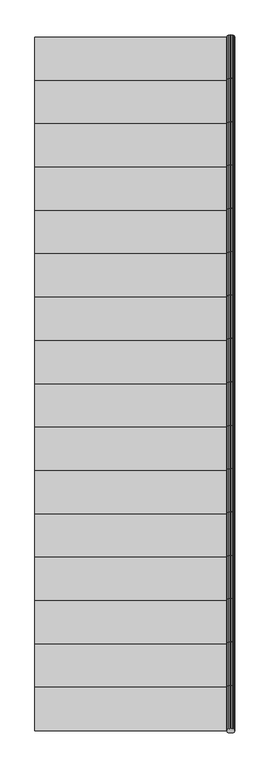
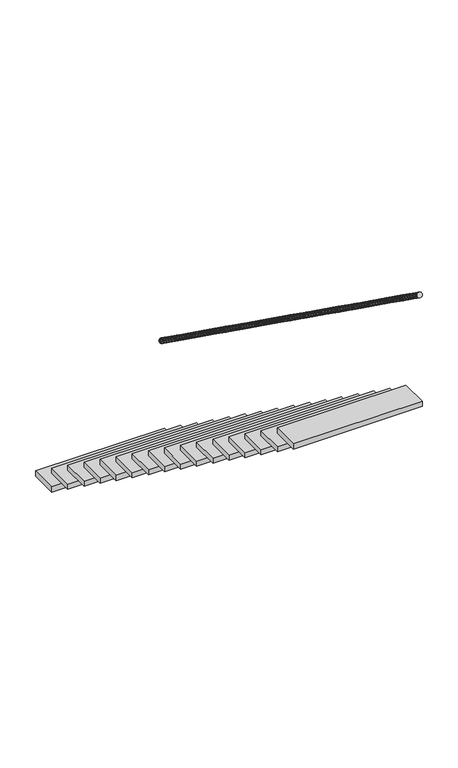
"""IFC4 building model written with IfcOpenShell, lengths in millimetres: stair geometry, 0_3d."""

from ifc_helpers import new_model, si_unit, frame, origin, origin_with_axes, place, context, project, spatial, polyline, outline, extrude, source, transform, mapped, element, save


def stair_085bacb0(model_context):
    return source(origin(), model_context, "Body", "SweptSolid", [
        extrude(outline(polyline([(1200.0, 3653.5347238), (1200.0, 3393.5347238), (0.0, 3393.5347238), (0.0, 3653.5347238), (1200.0, 3653.5347238)])), frame((0.0, 0.0, 371.7647059), z_axis=(0.0, 0.0, 1.0), x_axis=(1.0, 0.0, 0.0)), (0.0, 0.0, 1.0), 50.0),
        extrude(outline(polyline([(1200.0, 3913.5347238), (1200.0, 3653.5347238), (0.0, 3653.5347238), (0.0, 3913.5347238), (1200.0, 3913.5347238)])), frame((0.0, 0.0, 185.8823529), z_axis=(0.0, 0.0, 1.0), x_axis=(1.0, 0.0, 0.0)), (0.0, 0.0, 1.0), 50.0),
        extrude(outline(polyline([(1200.0, 793.5347238), (1200.0, 533.5347238), (0.0, 533.5347238), (0.0, 793.5347238), (1200.0, 793.5347238)])), frame((0.0, 0.0, 2416.4705882), z_axis=(0.0, 0.0, 1.0), x_axis=(1.0, 0.0, 0.0)), (0.0, 0.0, 1.0), 50.0),
        extrude(outline(polyline([(1.2235871, -7.1914682), (0.0, 0.0), (1.2235871, 7.1914683), (4.7745751, 13.6789856), (10.3053687, 18.8275083), (17.2745751, 22.1330636), (25.0, 23.2720803), (32.7254249, 22.1330636), (39.6946313, 18.8275083), (45.2254249, 13.6789856), (48.7764129, 7.1914683), (50.0, 0.0), (48.7764129, -7.1914682), (45.2254249, -13.6789855), (39.6946313, -18.8275083), (32.7254249, -22.1330635), (25.0, -23.2720801), (17.2745751, -22.1330635), (10.3053687, -18.8275083), (4.7745751, -13.6789855), (1.2235871, -7.1914682)])), frame((1150.0, 793.5347238, 3337.4705882), z_axis=(0.0, -0.8134846854821957, 0.5815863362269899), x_axis=(1.0, 0.0, 0.0)), (0.0, 0.0, 1.0), 319.6126548),
        extrude(outline(polyline([(1.2235871, -7.1914682), (0.0, 0.0), (1.2235871, 7.1914683), (4.7745751, 13.6789856), (10.3053687, 18.8275083), (17.2745751, 22.1330636), (25.0, 23.2720802), (32.7254249, 22.1330636), (39.6946313, 18.8275083), (45.2254249, 13.6789856), (48.7764129, 7.1914683), (50.0, 0.0), (48.7764129, -7.1914682), (45.2254249, -13.6789855), (39.6946313, -18.8275083), (32.7254249, -22.1330635), (25.0, -23.2720801), (17.2745751, -22.1330635), (10.3053687, -18.8275083), (4.7745751, -13.6789855), (1.2235871, -7.1914682)])), frame((1150.0, 2093.5347238, 2408.0588235), z_axis=(0.0, -0.8134846854821992, 0.5815863362269849), x_axis=(1.0, 0.0, 0.0)), (0.0, 0.0, 1.0), 319.6126548),
        extrude(outline(polyline([(1200.0, 2093.5347238), (1200.0, 1833.5347238), (0.0, 1833.5347238), (0.0, 2093.5347238), (1200.0, 2093.5347238)])), frame((0.0, 0.0, 1487.0588235), z_axis=(0.0, 0.0, 1.0), x_axis=(1.0, 0.0, 0.0)), (0.0, 0.0, 1.0), 50.0),
        extrude(outline(polyline([(1.2235871, -7.1914682), (0.0, 0.0), (1.2235871, 7.1914683), (4.7745751, 13.6789856), (10.3053687, 18.8275084), (17.2745751, 22.1330636), (25.0, 23.2720803), (32.7254249, 22.1330636), (39.6946313, 18.8275084), (45.2254249, 13.6789856), (48.7764129, 7.1914683), (50.0, 0.0), (48.7764129, -7.1914682), (45.2254249, -13.6789855), (39.6946313, -18.8275083), (32.7254249, -22.1330634), (25.0, -23.2720801), (17.2745751, -22.1330634), (10.3053687, -18.8275083), (4.7745751, -13.6789855), (1.2235871, -7.1914682)])), frame((1150.0, 2613.5347238, 2036.2941176), z_axis=(0.0, -0.8134846854822039, 0.5815863362269784), x_axis=(1.0, 0.0, 0.0)), (0.0, 0.0, 1.0), 319.6126548),
        extrude(outline(polyline([(1.2235871, -7.1914682), (0.0, 0.0), (1.2235871, 7.1914683), (4.7745751, 13.6789856), (10.3053687, 18.8275084), (17.2745751, 22.1330636), (25.0, 23.2720803), (32.7254249, 22.1330636), (39.6946313, 18.8275084), (45.2254249, 13.6789856), (48.7764129, 7.1914683), (50.0, 0.0), (48.7764129, -7.1914682), (45.2254249, -13.6789855), (39.6946313, -18.8275083), (32.7254249, -22.1330635), (25.0, -23.2720801), (17.2745751, -22.1330635), (10.3053687, -18.8275083), (4.7745751, -13.6789855), (1.2235871, -7.1914682)])), frame((1150.0, 3913.5347238, 1106.8823529), z_axis=(0.0, -0.8134846854822255, 0.5815863362269482), x_axis=(1.0, 0.0, 0.0)), (0.0, 0.0, 1.0), 319.6126548),
        extrude(outline(polyline([(1200.0, 1833.5347238), (1200.0, 1573.5347238), (0.0, 1573.5347238), (0.0, 1833.5347238), (1200.0, 1833.5347238)])), frame((0.0, 0.0, 1672.9411765), z_axis=(0.0, 0.0, 1.0), x_axis=(1.0, 0.0, 0.0)), (0.0, 0.0, 1.0), 50.0),
        extrude(outline(polyline([(1.2235871, -7.1914682), (0.0, 0.0), (1.2235871, 7.1914683), (4.7745751, 13.6789855), (10.3053687, 18.8275083), (17.2745751, 22.1330636), (25.0, 23.2720802), (32.7254249, 22.1330636), (39.6946313, 18.8275083), (45.2254249, 13.6789855), (48.7764129, 7.1914683), (50.0, 0.0), (48.7764129, -7.1914682), (45.2254249, -13.6789855), (39.6946313, -18.8275083), (32.7254249, -22.1330635), (25.0, -23.2720801), (17.2745751, -22.1330635), (10.3053687, -18.8275083), (4.7745751, -13.6789855), (1.2235871, -7.1914682)])), frame((1150.0, 533.5347238, 3523.3529412), z_axis=(0.0, -0.8134846854822048, 0.581586336226977), x_axis=(1.0, 0.0, 0.0)), (0.0, 0.0, 1.0), 319.6126548),
        extrude(outline(polyline([(1200.0, 1573.5347238), (1200.0, 1313.5347238), (0.0, 1313.5347238), (0.0, 1573.5347238), (1200.0, 1573.5347238)])), frame((0.0, 0.0, 1858.8235294), z_axis=(0.0, 0.0, 1.0), x_axis=(1.0, 0.0, 0.0)), (0.0, 0.0, 1.0), 50.0),
        extrude(outline(polyline([(1200.0, 2353.5347238), (1200.0, 2093.5347238), (0.0, 2093.5347238), (0.0, 2353.5347238), (1200.0, 2353.5347238)])), frame((0.0, 0.0, 1301.1764706), z_axis=(0.0, 0.0, 1.0), x_axis=(1.0, 0.0, 0.0)), (0.0, 0.0, 1.0), 50.0),
        extrude(outline(polyline([(1200.0, 533.5347238), (1200.0, 273.5347238), (0.0, 273.5347238), (0.0, 533.5347238), (1200.0, 533.5347238)])), frame((0.0, 0.0, 2602.3529412), z_axis=(0.0, 0.0, 1.0), x_axis=(1.0, 0.0, 0.0)), (0.0, 0.0, 1.0), 50.0),
        extrude(outline(polyline([(1.2235871, -7.1914682), (0.0, 0.0), (1.2235871, 7.1914683), (4.7745751, 13.6789855), (10.3053687, 18.8275083), (17.2745751, 22.1330636), (25.0, 23.2720802), (32.7254249, 22.1330636), (39.6946313, 18.8275083), (45.2254249, 13.6789855), (48.7764129, 7.1914683), (50.0, 0.0), (48.7764129, -7.1914682), (45.2254249, -13.6789855), (39.6946313, -18.8275083), (32.7254249, -22.1330635), (25.0, -23.2720801), (17.2745751, -22.1330635), (10.3053687, -18.8275083), (4.7745751, -13.6789855), (1.2235871, -7.1914682)])), frame((1150.0, 2873.5347238, 1850.4117647), z_axis=(0.0, -0.813484685482208, 0.5815863362269725), x_axis=(1.0, 0.0, 0.0)), (0.0, 0.0, 1.0), 319.6126548),
        extrude(outline(polyline([(1.2235871, -7.1914682), (0.0, 0.0), (1.2235871, 7.1914683), (4.7745751, 13.6789855), (10.3053687, 18.8275083), (17.2745751, 22.1330635), (25.0, 23.2720802), (32.7254249, 22.1330635), (39.6946313, 18.8275083), (45.2254249, 13.6789855), (48.7764129, 7.1914683), (50.0, 0.0), (48.7764129, -7.1914682), (45.2254249, -13.6789855), (39.6946313, -18.8275084), (32.7254249, -22.1330635), (25.0, -23.2720802), (17.2745751, -22.1330635), (10.3053687, -18.8275084), (4.7745751, -13.6789855), (1.2235871, -7.1914682)])), frame((1150.0, 1313.5347238, 2965.7058824), z_axis=(0.0, -0.81348468548223, 0.5815863362269419), x_axis=(1.0, 0.0, 0.0)), (0.0, 0.0, 1.0), 319.6126548),
        extrude(outline(polyline([(1.2235871, -7.1914682), (0.0, 0.0), (1.2235871, 7.1914683), (4.7745751, 13.6789855), (10.3053687, 18.8275083), (17.2745751, 22.1330636), (25.0, 23.2720802), (32.7254249, 22.1330636), (39.6946313, 18.8275083), (45.2254249, 13.6789855), (48.7764129, 7.1914683), (50.0, 0.0), (48.7764129, -7.1914682), (45.2254249, -13.6789855), (39.6946313, -18.8275083), (32.7254249, -22.1330635), (25.0, -23.2720801), (17.2745751, -22.1330635), (10.3053687, -18.8275083), (4.7745751, -13.6789855), (1.2235871, -7.1914682)])), frame((1150.0, 4173.5347238, 921.0), z_axis=(0.0, -0.8134846854822141, 0.5815863362269641), x_axis=(1.0, 0.0, 0.0)), (0.0, 0.0, 1.0), 319.6126548),
        extrude(outline(polyline([(1.2235871, -7.1914682), (0.0, 0.0), (1.2235871, 7.1914683), (4.7745751, 13.6789855), (10.3053687, 18.8275083), (17.2745751, 22.1330636), (25.0, 23.2720802), (32.7254249, 22.1330636), (39.6946313, 18.8275083), (45.2254249, 13.6789855), (48.7764129, 7.1914683), (50.0, 0.0), (48.7764129, -7.1914682), (45.2254249, -13.6789855), (39.6946313, -18.8275083), (32.7254249, -22.1330635), (25.0, -23.2720801), (17.2745751, -22.1330635), (10.3053687, -18.8275083), (4.7745751, -13.6789855), (1.2235871, -7.1914682)])), frame((1150.0, 273.5347238, 3709.2352941), z_axis=(0.0, -0.8134846854821822, 0.5815863362270085), x_axis=(1.0, 0.0, 0.0)), (0.0, 0.0, 1.0), 319.6126548),
        extrude(outline(polyline([(1200.0, 4173.5347238), (1200.0, 3913.5347238), (0.0, 3913.5347238), (0.0, 4173.5347238), (1200.0, 4173.5347238)])), origin_with_axes(), (0.0, 0.0, 1.0), 50.0),
        extrude(outline(polyline([(1200.0, 273.5347238), (1200.0, 13.5347238), (0.0, 13.5347238), (0.0, 273.5347238), (1200.0, 273.5347238)])), frame((0.0, 0.0, 2788.2352941), z_axis=(0.0, 0.0, 1.0), x_axis=(1.0, 0.0, 0.0)), (0.0, 0.0, 1.0), 50.0),
        extrude(outline(polyline([(1200.0, 3393.5347238), (1200.0, 3133.5347238), (0.0, 3133.5347238), (0.0, 3393.5347238), (1200.0, 3393.5347238)])), frame((0.0, 0.0, 557.6470588), z_axis=(0.0, 0.0, 1.0), x_axis=(1.0, 0.0, 0.0)), (0.0, 0.0, 1.0), 50.0),
        extrude(outline(polyline([(1.2235871, -7.1914682), (0.0, 0.0), (1.2235871, 7.1914683), (4.7745751, 13.6789856), (10.3053687, 18.8275083), (17.2745751, 22.1330636), (25.0, 23.2720802), (32.7254249, 22.1330636), (39.6946313, 18.8275083), (45.2254249, 13.6789856), (48.7764129, 7.1914683), (50.0, 0.0), (48.7764129, -7.1914682), (45.2254249, -13.6789855), (39.6946313, -18.8275083), (32.7254249, -22.1330635), (25.0, -23.2720801), (17.2745751, -22.1330635), (10.3053687, -18.8275083), (4.7745751, -13.6789855), (1.2235871, -7.1914682)])), frame((1150.0, 3393.5347238, 1478.6470588), z_axis=(0.0, -0.8134846854822252, 0.5815863362269487), x_axis=(1.0, 0.0, 0.0)), (0.0, 0.0, 1.0), 319.6126548),
        extrude(outline(polyline([(1.2235871, -7.1914682), (0.0, 0.0), (1.2235871, 7.1914683), (4.7745751, 13.6789855), (10.3053687, 18.8275083), (17.2745751, 22.1330636), (25.0, 23.2720802), (32.7254249, 22.1330636), (39.6946313, 18.8275083), (45.2254249, 13.6789855), (48.7764129, 7.1914683), (50.0, 0.0), (48.7764129, -7.1914682), (45.2254249, -13.6789855), (39.6946313, -18.8275083), (32.7254249, -22.1330635), (25.0, -23.2720801), (17.2745751, -22.1330635), (10.3053687, -18.8275083), (4.7745751, -13.6789855), (1.2235871, -7.1914682)])), frame((1150.0, 3653.5347238, 1292.7647059), z_axis=(0.0, -0.8134846854822023, 0.5815863362269806), x_axis=(1.0, 0.0, 0.0)), (0.0, 0.0, 1.0), 319.6126548),
        extrude(outline(polyline([(1200.0, 1053.5347238), (1200.0, 793.5347238), (0.0, 793.5347238), (0.0, 1053.5347238), (1200.0, 1053.5347238)])), frame((0.0, 0.0, 2230.5882353), z_axis=(0.0, 0.0, 1.0), x_axis=(1.0, 0.0, 0.0)), (0.0, 0.0, 1.0), 50.0),
        extrude(outline(polyline([(1.2235871, -7.1914682), (0.0, 0.0), (1.2235871, 7.1914683), (4.7745751, 13.6789855), (10.3053687, 18.8275083), (17.2745751, 22.1330636), (25.0, 23.2720802), (32.7254249, 22.1330636), (39.6946313, 18.8275083), (45.2254249, 13.6789855), (48.7764129, 7.1914683), (50.0, 0.0), (48.7764129, -7.1914682), (45.2254249, -13.6789855), (39.6946313, -18.8275083), (32.7254249, -22.1330635), (25.0, -23.2720801), (17.2745751, -22.1330635), (10.3053687, -18.8275083), (4.7745751, -13.6789855), (1.2235871, -7.1914682)])), frame((1150.0, 2353.5347238, 2222.1764706), z_axis=(0.0, -0.8134846854822106, 0.5815863362269689), x_axis=(1.0, 0.0, 0.0)), (0.0, 0.0, 1.0), 319.6126548),
        extrude(outline(polyline([(1200.0, 2873.5347238), (1200.0, 2613.5347238), (0.0, 2613.5347238), (0.0, 2873.5347238), (1200.0, 2873.5347238)])), frame((0.0, 0.0, 929.4117647), z_axis=(0.0, 0.0, 1.0), x_axis=(1.0, 0.0, 0.0)), (0.0, 0.0, 1.0), 50.0),
        extrude(outline(polyline([(1200.0, 1313.5347238), (1200.0, 1053.5347238), (0.0, 1053.5347238), (0.0, 1313.5347238), (1200.0, 1313.5347238)])), frame((0.0, 0.0, 2044.7058824), z_axis=(0.0, 0.0, 1.0), x_axis=(1.0, 0.0, 0.0)), (0.0, 0.0, 1.0), 50.0),
        extrude(outline(polyline([(1.2235871, -7.1914682), (0.0, 0.0), (1.2235871, 7.1914683), (4.7745751, 13.6789855), (10.3053687, 18.8275083), (17.2745751, 22.1330636), (25.0, 23.2720802), (32.7254249, 22.1330636), (39.6946313, 18.8275083), (45.2254249, 13.6789855), (48.7764129, 7.1914683), (50.0, 0.0), (48.7764129, -7.1914682), (45.2254249, -13.6789855), (39.6946313, -18.8275083), (32.7254249, -22.1330635), (25.0, -23.2720801), (17.2745751, -22.1330635), (10.3053687, -18.8275083), (4.7745751, -13.6789855), (1.2235871, -7.1914682)])), frame((1150.0, 1833.5347238, 2593.9411765), z_axis=(0.0, -0.8134846854822316, 0.5815863362269396), x_axis=(1.0, 0.0, 0.0)), (0.0, 0.0, 1.0), 319.6126548),
        extrude(outline(polyline([(1.2235871, -7.1914682), (0.0, 0.0), (1.2235871, 7.1914683), (4.7745751, 13.6789855), (10.3053687, 18.8275083), (17.2745751, 22.1330636), (25.0, 23.2720802), (32.7254249, 22.1330636), (39.6946313, 18.8275083), (45.2254249, 13.6789855), (48.7764129, 7.1914683), (50.0, 0.0), (48.7764129, -7.1914682), (45.2254249, -13.6789855), (39.6946313, -18.8275083), (32.7254249, -22.1330635), (25.0, -23.2720802), (17.2745751, -22.1330635), (10.3053687, -18.8275083), (4.7745751, -13.6789855), (1.2235871, -7.1914682)])), frame((1150.0, 3133.5347238, 1664.5294118), z_axis=(0.0, -0.813484685482228, 0.5815863362269446), x_axis=(1.0, 0.0, 0.0)), (0.0, 0.0, 1.0), 319.6126548),
        extrude(outline(polyline([(1200.0, 3133.5347238), (1200.0, 2873.5347238), (0.0, 2873.5347238), (0.0, 3133.5347238), (1200.0, 3133.5347238)])), frame((0.0, 0.0, 743.5294118), z_axis=(0.0, 0.0, 1.0), x_axis=(1.0, 0.0, 0.0)), (0.0, 0.0, 1.0), 50.0),
        extrude(outline(polyline([(1200.0, 2613.5347238), (1200.0, 2353.5347238), (0.0, 2353.5347238), (0.0, 2613.5347238), (1200.0, 2613.5347238)])), frame((0.0, 0.0, 1115.2941176), z_axis=(0.0, 0.0, 1.0), x_axis=(1.0, 0.0, 0.0)), (0.0, 0.0, 1.0), 50.0),
        extrude(outline(polyline([(1.2235871, -7.1914682), (0.0, 0.0), (1.2235871, 7.1914683), (4.7745751, 13.6789855), (10.3053687, 18.8275083), (17.2745751, 22.1330636), (25.0, 23.2720802), (32.7254249, 22.1330636), (39.6946313, 18.8275083), (45.2254249, 13.6789855), (48.7764129, 7.1914683), (50.0, 0.0), (48.7764129, -7.1914682), (45.2254249, -13.6789855), (39.6946313, -18.8275083), (32.7254249, -22.1330635), (25.0, -23.2720801), (17.2745751, -22.1330635), (10.3053687, -18.8275083), (4.7745751, -13.6789855), (1.2235871, -7.1914682)])), frame((1150.0, 1573.5347238, 2779.8235294), z_axis=(0.0, -0.8134846854822146, 0.5815863362269632), x_axis=(1.0, 0.0, 0.0)), (0.0, 0.0, 1.0), 319.6126548),
        extrude(outline(polyline([(1.2235871, -7.1914682), (0.0, 0.0), (1.2235871, 7.1914683), (4.7745751, 13.6789855), (10.3053687, 18.8275083), (17.2745751, 22.1330636), (25.0, 23.2720802), (32.7254249, 22.1330636), (39.6946313, 18.8275083), (45.2254249, 13.6789855), (48.7764129, 7.1914683), (50.0, 0.0), (48.7764129, -7.1914682), (45.2254249, -13.6789855), (39.6946313, -18.8275083), (32.7254249, -22.1330635), (25.0, -23.2720801), (17.2745751, -22.1330635), (10.3053687, -18.8275083), (4.7745751, -13.6789855), (1.2235871, -7.1914682)])), frame((1150.0, 1053.5347238, 3151.5882353), z_axis=(0.0, -0.8134846854821998, 0.5815863362269841), x_axis=(1.0, 0.0, 0.0)), (0.0, 0.0, 1.0), 319.6126548),
    ])


if __name__ == "__main__":
    model = new_model("IFC4")
    model_context = context("Model", 3, world=origin())
    ifc_project = project(units=[si_unit("LENGTHUNIT", "METRE", prefix="MILLI")], contexts=[model_context])
    site = spatial("IfcSite", under=ifc_project)
    building = spatial("IfcBuilding", under=site)
    placement = place(None, origin())
    stair_shape = stair_085bacb0(model_context)
    element("IfcStair", 1, ObjectType="0_3d", at=placement, inside=building, context=model_context, shape_type="MappedRepresentation", body=[
        mapped(stair_shape, transform((0.0, 0.0, 0.0), x_axis=(1.0, 0.0, 0.0), y_axis=(0.0, 1.0, 0.0), z_axis=(0.0, 0.0, 1.0))),
    ])
    save(model, "model.ifc")

# Revit data of these elements
# Element 1 (IfcStair, "0_3d")
#   Materials on its faces: "*1", "weiss"
# Materials
#   "*1": class "Unassigned", colour RGB 175 175 175, transparency 0
#   "weiss": class "Unassigned", colour RGB 255 255 255, transparency 0
